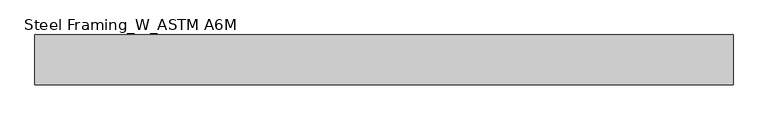
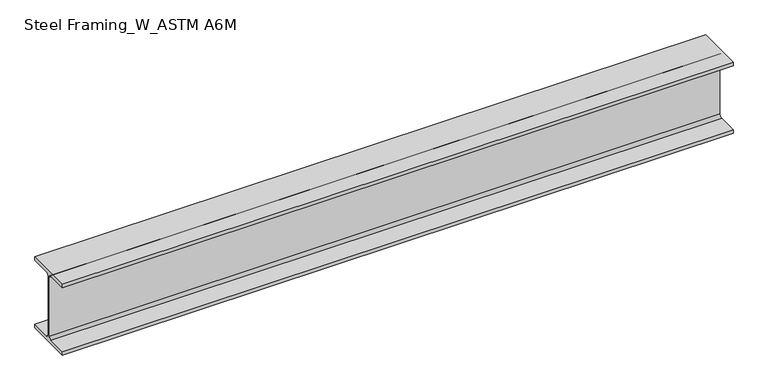
"""IFC4 building model written with IfcOpenShell, lengths in millimetres: beam geometry, Steel Framing_W_ASTM A6M : H_SB_AR_S02_W200x31.3_B6."""

from ifc_helpers import new_model, si_unit, point, frame, frame_2d, origin, place, context, project, spatial, polyline, circle_curve, trimmed, segment, composite_curve, outline, extrude, source, transform, mapped, element, save


def steel_framing_w_astm_a6m_9f2baa18(model_context):
    return source(origin(), model_context, "Body", "SweptSolid", [
        extrude(outline(composite_curve([segment(polyline([(67.0, -94.8), (67.0, -105.0), (-67.0, -105.0), (-67.0, -94.8), (-10.775, -94.8)]), True, "CONTINUOUS"), segment(trimmed(circle_curve(frame_2d((-10.775, -87.2)), 7.6), [point((-10.775, -94.8))], [point((-3.175, -87.2))], True, "CARTESIAN"), True, "CONTINUOUS"), segment(polyline([(-3.175, -87.2), (-3.175, 87.2)]), True, "CONTINUOUS"), segment(trimmed(circle_curve(frame_2d((-10.775, 87.2)), 7.6), [point((-3.175, 87.2))], [point((-10.775, 94.8))], True, "CARTESIAN"), True, "CONTINUOUS"), segment(polyline([(-10.775, 94.8), (-67.0, 94.8), (-67.0, 105.0), (67.0, 105.0), (67.0, 94.8), (10.775, 94.8)]), True, "CONTINUOUS"), segment(trimmed(circle_curve(frame_2d((10.775, 87.2)), 7.6), [point((10.775, 94.8))], [point((3.175, 87.2))], True, "CARTESIAN"), True, "CONTINUOUS"), segment(polyline([(3.175, 87.2), (3.175, -87.2)]), True, "CONTINUOUS"), segment(trimmed(circle_curve(frame_2d((10.775, -87.2)), 7.6), [point((3.175, -87.2))], [point((10.775, -94.8))], True, "CARTESIAN"), True, "CONTINUOUS"), segment(polyline([(10.775, -94.8), (67.0, -94.8)]), True, "CONTINUOUS")], self_intersect=False)), frame((-985.55, 0.0, 0.0), z_axis=(1.0, 0.0, 0.0), x_axis=(0.0, 1.0, 0.0)), (0.0, 0.0, 1.0), 1883.4),
    ])


if __name__ == "__main__":
    model = new_model("IFC4")
    model_context = context("Model", 3, world=origin())
    ifc_project = project(units=[si_unit("LENGTHUNIT", "METRE", prefix="MILLI")], contexts=[model_context])
    site = spatial("IfcSite", under=ifc_project)
    building = spatial("IfcBuilding", under=site)
    placement = place(None, origin())
    steel_framing_w_astm_a6m_shape = steel_framing_w_astm_a6m_9f2baa18(model_context)
    element("IfcBeam", 1, ObjectType="Steel Framing_W_ASTM A6M : H_SB_AR_S02_W200x31.3_B6", at=placement, inside=building, context=model_context, shape_type="MappedRepresentation", body=[
        mapped(steel_framing_w_astm_a6m_shape, transform((0.0, 0.0, 0.0), x_axis=(1.0, 0.0, 0.0), y_axis=(0.0, 1.0, 0.0), z_axis=(0.0, 0.0, 1.0))),
    ])
    save(model, "model.ifc")

# Revit data of these elements
# Type "Steel Framing_W_ASTM A6M : H_SB_AR_S02_W200x31.3_B6"
#   Type Mark = "B6"
#   Section Name Key = "W8x21"
#   Width = 13.4 cm
#   Web Thickness = 0.635 cm
#   Web Fillet = 0.76 cm
#   Warping Constant = 40800.0 cm⁶
#   Torsional Moment of Inertia = 11.70 cm⁴
#   Section Area = 39.7 cm²
#   Plastic Modulus weak axis = 93.2 cm³
#   Plastic Modulus strong axis = 334.0 cm³
#   Perimeter = 0.93 m²/m
#   Nominal Weight = 31.30 kgf/m
#   Moment of Inertia weak axis = 407.00 cm⁴
#   Moment of Inertia strong axis = 3130.00 cm⁴
#   Height = 21.0 cm
#   Flange Thickness = 1.02 cm
#   Elastic Modulus weak axis = 60.8 cm³
#   Elastic Modulus strong axis = 298.0 cm³
#   Centroid Vertical = 10.5 cm
#   Centroid Horizontal = 6.7 cm
#   Length [instance default] = 1500 mm
#   Structural Material [instance default] = Steel, 45-345
#   Bolt Spacing = 0
#   Assembly Code = ""
# Element 1 (IfcBeam, "Steel Framing_W_ASTM A6M : H_SB_AR_S02_W200x31.3_B6")
#   Materials on its faces: "Steel, 45-345"
# Materials
#   "Steel, 45-345": class "Metal", colour RGB 189 187 185, transparency 0, Description = "Steel 345 MPa", Cost = 0
